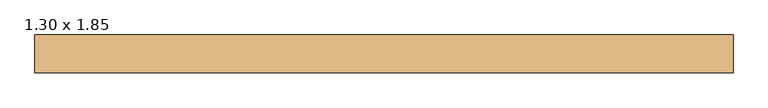
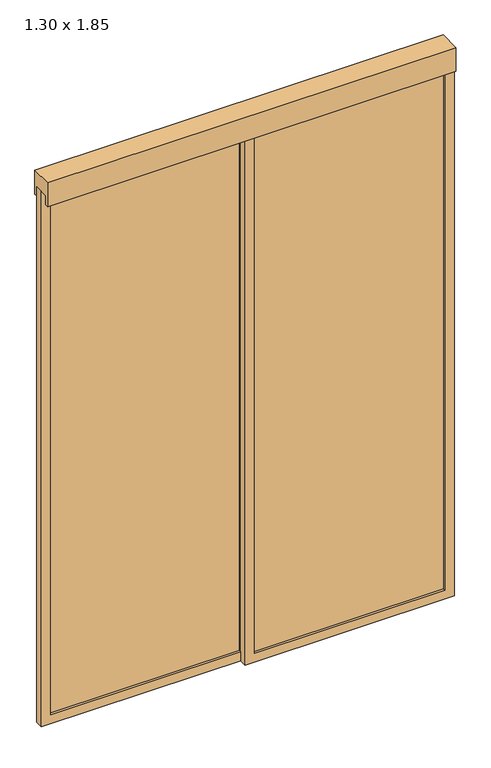
"""IFC4 building model written with IfcOpenShell, lengths in millimetres: door geometry, CC_BOX VIDRO RETO : 1.30 x 1.85."""

from ifc_helpers import new_model, si_unit, frame, origin, place, context, project, spatial, polyline, outline, extrude, source, transform, mapped, element, save


def door_1_30_x_1_85_e645ec63(model_context):
    return source(origin(), model_context, "Body", "SweptSolid", [
        extrude(outline(polyline([(620.0, -7.5), (620.0, -17.5), (15.0, -17.5), (15.0, -7.5), (620.0, -7.5)])), frame((0.0, 0.0, 30.0), z_axis=(0.0, 0.0, 1.0), x_axis=(1.0, 0.0, 0.0)), (0.0, 0.0, 1.0), 1740.0),
        extrude(outline(polyline([(1800.0, 650.0), (1800.0, -15.0), (0.0, -15.0), (0.0, 650.0), (1800.0, 650.0)]), holes=[polyline([(1770.0, 620.0), (30.0, 620.0), (30.0, 15.0), (1770.0, 15.0), (1770.0, 620.0)])]), frame((0.0, -25.0, 0.0), z_axis=(0.0, 1.0, 0.0), x_axis=(0.0, 0.0, 1.0)), (0.0, 0.0, 1.0), 25.0),
        extrude(outline(polyline([(-15.0, 17.5), (-15.0, 7.5), (-620.0, 7.5), (-620.0, 17.5), (-15.0, 17.5)])), frame((0.0, 0.0, 30.0), z_axis=(0.0, 0.0, 1.0), x_axis=(1.0, 0.0, 0.0)), (0.0, 0.0, 1.0), 1740.0),
        extrude(outline(polyline([(1800.0, 15.0), (1800.0, -650.0), (0.0, -650.0), (0.0, 15.0), (1800.0, 15.0)]), holes=[polyline([(1770.0, -15.0), (30.0, -15.0), (30.0, -620.0), (1770.0, -620.0), (1770.0, -15.0)])]), frame((0.0, 0.0, 0.0), z_axis=(0.0, 1.0, 0.0), x_axis=(0.0, 0.0, 1.0)), (0.0, 0.0, 1.0), 25.0),
        extrude(outline(polyline([(25.0, 1800.0), (-25.0, 1800.0), (-25.0, 1770.0), (-35.0, 1770.0), (-35.0, 1850.0), (35.0, 1850.0), (35.0, 1770.0), (25.0, 1770.0), (25.0, 1800.0)])), frame((-650.0, 0.0, 0.0), z_axis=(1.0, 0.0, 0.0), x_axis=(0.0, 1.0, 0.0)), (0.0, 0.0, 1.0), 1300.0),
    ])


if __name__ == "__main__":
    model = new_model("IFC4")
    model_context = context("Model", 3, world=origin())
    ifc_project = project(units=[si_unit("LENGTHUNIT", "METRE", prefix="MILLI")], contexts=[model_context])
    site = spatial("IfcSite", under=ifc_project)
    building = spatial("IfcBuilding", under=site)
    placement = place(None, origin())
    door_1_30_x_1_85_shape = door_1_30_x_1_85_e645ec63(model_context)
    element("IfcDoor", 1, ObjectType="CC_BOX VIDRO RETO : 1.30 x 1.85", at=placement, inside=building, context=model_context, shape_type="MappedRepresentation", body=[
        mapped(door_1_30_x_1_85_shape, transform((0.0, 0.0, 0.0), x_axis=(1.0, 0.0, 0.0), y_axis=(0.0, 1.0, 0.0), z_axis=(0.0, 0.0, 1.0))),
    ])
    save(model, "model.ifc")

# Revit data of these elements
# Type "CC_BOX VIDRO RETO : 1.30 x 1.85"
#   Type Mark = "BOX"
#   Site = "www.construir.arq.br"
#   Empresa = "Cursos Construir"
#   Criado Por = "Roberto Netto"
#   Analytic Construction = "<Nenhum>"
#   Atualizado por = "Rudemberg Eloi"
#   Rough Width = 1.30 m
#   Largura Moldura [instance default] = 0.03 m
#   Largura Folha [instance default] = 0.665 m
#   Width = 1.30 m
#   Espessura Vidro [instance default] = 0.01 m
#   Espessura Folha [instance default] = 0.025 m
#   Thickness = 0.05 m
#   Rough Height = 1.85 m
#   Altura Folha [instance default] = 1.80 m
#   Height = 1.85 m
#   ----FOLHA---- [instance default] = 0.00 m
#   Material Vidro = .VIDRO
#   Material Trilho = .ALUMÍNIO COM PINTURA ELETROSTÁTICA BRANCA
#   Material Moldura = .ALUMÍNIO COM PINTURA ELETROSTÁTICA BRANCA
#   Function = (empty or 0)
#   Description = (empty or 0)
# Element 1 (IfcDoor, "CC_BOX VIDRO RETO : 1.30 x 1.85")
#   Materials on its faces: ".ALUMÍNIO COM PINTURA ELETROSTÁTICA BRANCA", ".VIDRO"
# Materials
#   ".VIDRO": class "Genérico", colour RGB 198 236 255, transparency 0.95, Cost = 0
#   ".ALUMÍNIO COM PINTURA ELETROSTÁTICA BRANCA": class "CC_METAIS", colour RGB 241 241 241, transparency 0, Cost = 0
